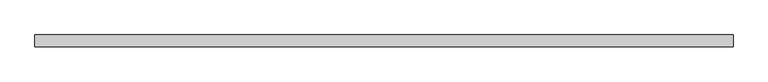
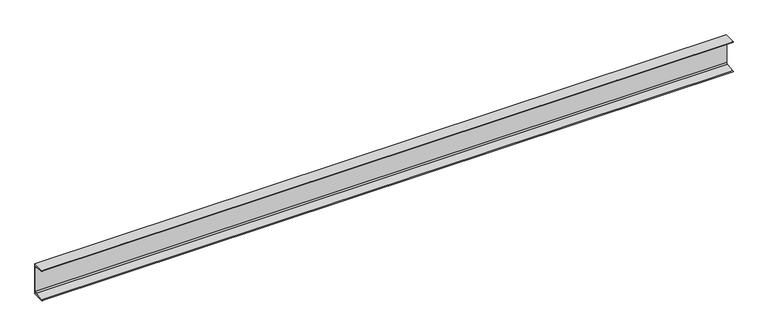
"""IFC4 building model written with IfcOpenShell, lengths in millimetres: beam geometry, C-образный профиль (ГОСТ 8240-89) Балки : [ 22."""

from ifc_helpers import new_model, si_unit, point, frame, frame_2d, origin, place, context, project, spatial, polyline, circle_curve, trimmed, segment, composite_curve, outline, extrude, source, transform, mapped, element, save


def beam_ce67fa95(model_context):
    return source(origin(), model_context, "Body", "SweptSolid", [
        extrude(outline(composite_curve([segment(polyline([(22.1, 110.0), (22.1, -110.0), (-59.9, -110.0), (-59.9, -108.9686971)]), True, "CONTINUOUS"), segment(trimmed(circle_curve(frame_2d((-55.9, -108.9686971)), 4.0), [point((-59.9, -108.9686971))], [point((-56.3765809, -104.9971897))], False, "CARTESIAN"), True, "CONTINUOUS"), segment(polyline([(-56.3765809, -104.9971897), (7.8914522, -97.2850257)]), True, "CONTINUOUS"), segment(trimmed(circle_curve(frame_2d((6.7, -87.3562574)), 10.0), [point((7.8914522, -97.2850257))], [point((16.7, -87.3562574))], True, "CARTESIAN"), True, "CONTINUOUS"), segment(polyline([(16.7, -87.3562574), (16.7, 87.3562574)]), True, "CONTINUOUS"), segment(trimmed(circle_curve(frame_2d((6.7, 87.3562574)), 10.0), [point((16.7, 87.3562574))], [point((7.8914522, 97.2850257))], True, "CARTESIAN"), True, "CONTINUOUS"), segment(polyline([(7.8914522, 97.2850257), (-56.3765809, 104.9971897)]), True, "CONTINUOUS"), segment(trimmed(circle_curve(frame_2d((-55.9, 108.9686971)), 4.0), [point((-56.3765809, 104.9971897))], [point((-59.9, 108.9686971))], False, "CARTESIAN"), True, "CONTINUOUS"), segment(polyline([(-59.9, 108.9686971), (-59.9, 110.0), (22.1, 110.0)]), True, "CONTINUOUS")], self_intersect=False)), frame((-2395.0, 0.0, 0.0), z_axis=(1.0, 0.0, 0.0), x_axis=(0.0, 1.0, 0.0)), (0.0, 0.0, 1.0), 4790.0),
    ])


if __name__ == "__main__":
    model = new_model("IFC4")
    model_context = context("Model", 3, world=origin())
    ifc_project = project(units=[si_unit("LENGTHUNIT", "METRE", prefix="MILLI")], contexts=[model_context])
    site = spatial("IfcSite", under=ifc_project)
    building = spatial("IfcBuilding", under=site)
    placement = place(None, origin())
    beam_shape = beam_ce67fa95(model_context)
    element("IfcBeam", 1, ObjectType="C-образный профиль (ГОСТ 8240-89) Балки : [ 22", at=placement, inside=building, context=model_context, shape_type="MappedRepresentation", body=[
        mapped(beam_shape, transform((0.0, 0.0, 0.0), x_axis=(1.0, 0.0, 0.0), y_axis=(0.0, 1.0, 0.0), z_axis=(0.0, 0.0, 1.0))),
    ])
    save(model, "model.ifc")

# Revit data of these elements
# Type "C-образный профиль (ГОСТ 8240-89) Балки : [ 22"
#   tf = 9.5 mm
#   ri = 4 mm
#   ra = 10 mm
#   W = 0.20594
#   Vz = 110 mm
#   Vy = 59.9 mm
#   Vpz = 110 mm
#   Vpy = 22.1 mm
#   Уклон = 0.12
#   Length [instance default] = 1500 mm
#   bf = 82 mm
#   d = 220 mm
#   tw = 5.4 mm
#   A = 0.00267 m²
#   Structural Material [instance default] = Металл - Сталь - 345 МПa
#   Assembly Code = ""
# Element 1 (IfcBeam, "C-образный профиль (ГОСТ 8240-89) Балки : [ 22")
#   Structural Material = C235
#   Materials on its faces: "C235"
# Materials
#   "Металл - Сталь - 345 МПa": class "Металл", colour RGB 247 247 247, transparency 0
#   "C235": class "Не назначено", colour RGB 0 0 0, transparency 0
